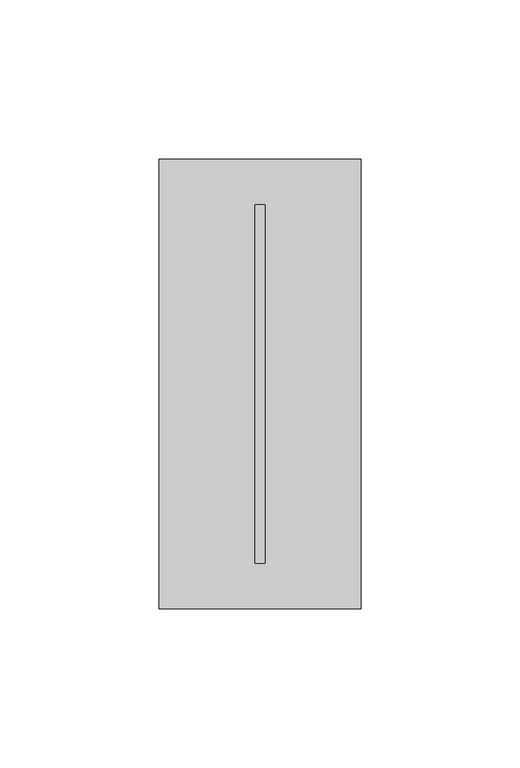
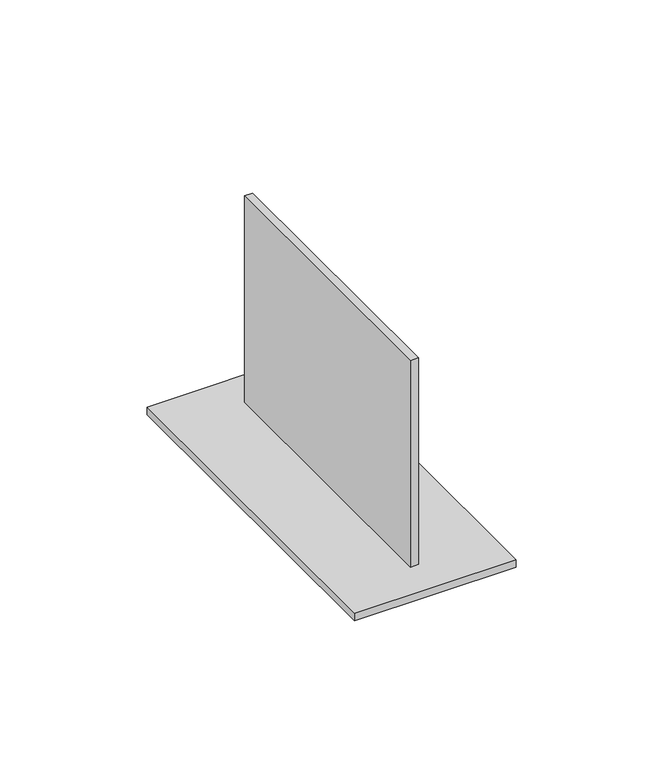
"""IFC4 building model written with IfcOpenShell, lengths in millimetres: proxy geometry, 060523 - W_P_C - Fastenings - Concealed Joist Ties : 060523 - W_P_C - Fastenings - Concealed Joist Ties."""

import ifcopenshell
import ifcopenshell.guid

model = None  # the IFC model being written
_history = None  # IfcOwnerHistory: only IFC2X3 demands one
_inside = {}  # id of a spatial element -> (the spatial element, [elements in it])
_under = {}  # id of a project, library or spatial element -> (it, [spatial elements below it])
_declared = {}  # id of a project -> (the project, [libraries it declares])
_typed = {}  # id of a type object -> (the type object, [elements of that type])
_made_of = {}  # id of a material, layer set ... -> (it, [elements and type objects made of it])


def new_model(schema):
    """Start an empty IFC model of exactly this schema.

    Asked for "IFC4X3", IfcOpenShell would pick the latest addendum, in which some entities
    have other attributes; the version numbers below select the first issue.
    IFC2X3 requires an IfcOwnerHistory on every rooted entity: one is made here for all.
    """
    global model, _history
    if schema == "IFC4X3":
        model = ifcopenshell.file(schema_version=(4, 3, 0, 0))
    else:
        model = ifcopenshell.file(schema=schema)
    _inside.clear()
    _under.clear()
    _declared.clear()
    _typed.clear()
    _made_of.clear()
    _history = None
    if model.schema == "IFC2X3":
        org = make("IfcOrganization", Name="unknown")
        user = make(
            "IfcPersonAndOrganization",
            ThePerson=make("IfcPerson", FamilyName="unknown"),
            TheOrganization=org,
        )
        app = make(
            "IfcApplication",
            ApplicationDeveloper=org,
            Version="unknown",
            ApplicationFullName="unknown",
            ApplicationIdentifier="unknown",
        )
        _history = make(
            "IfcOwnerHistory",
            OwningUser=user,
            OwningApplication=app,
            ChangeAction="ADDED",
            CreationDate=0,
        )
    return model


def make(cls, **values):
    """One entity of the class cls with the attributes given. An attribute that is None is left unset."""
    return model.create_entity(
        cls, **{name: value for name, value in values.items() if value is not None}
    )


def rooted(cls, **values):
    """An entity with a GlobalId (a new one), such as an element, a storey or a relation."""
    return make(cls, GlobalId=ifcopenshell.guid.new(), OwnerHistory=_history, **values)


def si_unit(unit_type, name, prefix=None):
    """IfcSIUnit, for example si_unit("LENGTHUNIT", "METRE", prefix="MILLI")."""
    return make("IfcSIUnit", UnitType=unit_type, Prefix=prefix, Name=name)


def assignment(units):
    """IfcUnitAssignment: the units of a project."""
    return None if units is None else make("IfcUnitAssignment", Units=units)


def point(xyz):
    """IfcCartesianPoint."""
    return None if xyz is None else make("IfcCartesianPoint", Coordinates=xyz)


def direction(xyz):
    """IfcDirection."""
    return None if xyz is None else make("IfcDirection", DirectionRatios=xyz)


def frame(location, z_axis=None, x_axis=None):
    """IfcAxis2Placement3D, a coordinate frame: its origin and axes. An axis left out is left unset."""
    return make(
        "IfcAxis2Placement3D",
        Location=point(location),
        Axis=direction(z_axis),
        RefDirection=direction(x_axis),
    )


def origin():
    """The frame at (0, 0, 0) with its axes left unset."""
    return frame((0.0, 0.0, 0.0))


def origin_with_axes():
    """The frame at (0, 0, 0) with the z axis (0, 0, 1) and the x axis (1, 0, 0) written out."""
    return frame((0.0, 0.0, 0.0), z_axis=(0.0, 0.0, 1.0), x_axis=(1.0, 0.0, 0.0))


def place(relative_to, where):
    """IfcLocalPlacement: puts the frame where relative to a parent placement (None: the world)."""
    return make(
        "IfcLocalPlacement", PlacementRelTo=relative_to, RelativePlacement=where
    )


def context(
    kind, dimensions, precision=None, world=None, true_north=None, identifier=None
):
    """IfcGeometricRepresentationContext, for example the 3D "Model" context."""
    return make(
        "IfcGeometricRepresentationContext",
        ContextIdentifier=identifier,
        ContextType=kind,
        CoordinateSpaceDimension=dimensions,
        Precision=precision,
        WorldCoordinateSystem=world,
        TrueNorth=true_north,
    )


def project(units=None, contexts=None):
    """IfcProject with its units and contexts."""
    return rooted(
        "IfcProject",
        Name="project",
        RepresentationContexts=contexts,
        UnitsInContext=assignment(units),
    )


def spatial(cls, under=None, at=None, **own):
    """A site, building, storey or space (cls), placed at a placement, below another one or the project."""
    s = rooted(cls, ObjectPlacement=at, **own)
    if under is not None:
        _under.setdefault(under.id(), (under, []))[1].append(s)
    return s


def polyline(points):
    """IfcPolyline through the points."""
    return make("IfcPolyline", Points=[point(p) for p in points])


def outline(outer, holes=None, kind="AREA"):
    """IfcArbitraryClosedProfileDef: a profile drawn as a closed curve; with holes, ...WithVoids."""
    if holes is None:
        return make("IfcArbitraryClosedProfileDef", ProfileType=kind, OuterCurve=outer)
    return make(
        "IfcArbitraryProfileDefWithVoids",
        ProfileType=kind,
        OuterCurve=outer,
        InnerCurves=holes,
    )


def extrude(swept, where, along, depth):
    """IfcExtrudedAreaSolid: the profile swept, set in the frame where, extruded along a direction by depth."""
    return make(
        "IfcExtrudedAreaSolid",
        SweptArea=swept,
        Position=where,
        ExtrudedDirection=direction(along),
        Depth=depth,
    )


def shape(context_of_items, identifier, shape_type, items):
    """IfcShapeRepresentation: the items that make up one representation, for example the "Body"."""
    return make(
        "IfcShapeRepresentation",
        ContextOfItems=context_of_items,
        RepresentationIdentifier=identifier,
        RepresentationType=shape_type,
        Items=items,
    )


def source(mapping_origin, context_of_items, identifier, shape_type, items):
    """IfcRepresentationMap: a shape defined once, which mapped items show again and again."""
    return make(
        "IfcRepresentationMap",
        MappingOrigin=mapping_origin,
        MappedRepresentation=shape(context_of_items, identifier, shape_type, items),
    )


def transform(
    local_origin,
    x_axis=None,
    y_axis=None,
    z_axis=None,
    scale=None,
    scale2=None,
    scale3=None,
    uniform=True,
):
    """IfcCartesianTransformationOperator3D, or its non-uniform kind. x_axis, y_axis, z_axis: its Axis1, 2, 3."""
    if uniform:
        return make(
            "IfcCartesianTransformationOperator3D",
            Axis1=direction(x_axis),
            Axis2=direction(y_axis),
            LocalOrigin=point(local_origin),
            Scale=scale,
            Axis3=direction(z_axis),
        )
    return make(
        "IfcCartesianTransformationOperator3DnonUniform",
        Axis1=direction(x_axis),
        Axis2=direction(y_axis),
        LocalOrigin=point(local_origin),
        Scale=scale,
        Axis3=direction(z_axis),
        Scale2=scale2,
        Scale3=scale3,
    )


def mapped(mapping_source, mapping_target):
    """IfcMappedItem: shows the shape of a source again, moved by a transform."""
    return make(
        "IfcMappedItem", MappingSource=mapping_source, MappingTarget=mapping_target
    )


def made_of(thing, what):
    """Note that an element or type object is made of a material, layer set ...; save() writes the relation."""
    if what is not None:
        _made_of.setdefault(what.id(), (what, []))[1].append(thing)
    return thing


def element(
    cls,
    number,
    at=None,
    inside=None,
    cuts=None,
    type_object=None,
    material=None,
    context=None,
    identifier="Body",
    shape_type=None,
    held_by="IfcProductDefinitionShape",
    body=None,
    shapes=None,
    **own,
):
    """One element of the class cls, such as IfcWall. Its Tag is "e" and its number.

    at: its placement. inside: the storey or other place that contains it. cuts: it is an
    opening in that element (IfcRelVoidsElement). A single representation is given by context,
    identifier, shape_type and body (its items); several are given by shapes. held_by: the class
    of the entity that holds the representations. save() writes the other relations.
    """
    e = rooted(cls, Tag="e%d" % number, ObjectPlacement=at, **own)
    if body is not None:
        shapes = [shape(context, identifier, shape_type, body)]
    if shapes is not None:
        e.Representation = make(held_by, Representations=shapes)
    if inside is not None:
        _inside.setdefault(inside.id(), (inside, []))[1].append(e)
    if cuts is not None:
        rooted(
            "IfcRelVoidsElement", RelatingBuildingElement=cuts, RelatedOpeningElement=e
        )
    if type_object is not None:
        _typed.setdefault(type_object.id(), (type_object, []))[1].append(e)
    return made_of(e, material)


def aggregate(whole, parts):
    """IfcRelAggregates: a whole, such as a stair, and the parts it consists of."""
    return rooted("IfcRelAggregates", RelatingObject=whole, RelatedObjects=parts)


def save(model, path):
    """Write the relations noted so far, then the file.

    IfcRelAggregates (storeys below a building ...), IfcRelContainedInSpatialStructure (elements
    in a storey), IfcRelDefinesByType, IfcRelAssociatesMaterial and IfcRelDeclares: one each for
    every whole, place, type object, material and project.
    """
    for whole, parts in _under.values():
        aggregate(whole, parts)
    for where, things in _inside.values():
        rooted(
            "IfcRelContainedInSpatialStructure",
            RelatedElements=things,
            RelatingStructure=where,
        )
    for kind, things in _typed.values():
        rooted("IfcRelDefinesByType", RelatedObjects=things, RelatingType=kind)
    for what, things in _made_of.values():
        rooted("IfcRelAssociatesMaterial", RelatedObjects=things, RelatingMaterial=what)
    for by, libraries in _declared.values():
        rooted("IfcRelDeclares", RelatingContext=by, RelatedDefinitions=libraries)
    model.write(path)


def generic_models_a2696cd2(model_context):
    return source(origin(), model_context, "Body", "SweptSolid", [
        extrude(outline(polyline([(1.5875, 56.35625), (1.5875, -56.35625), (-1.5875, -56.35625), (-1.5875, 56.35625), (1.5875, 56.35625)])), frame((0.0, 0.0, 3.175), z_axis=(0.0, 0.0, 1.0), x_axis=(1.0, 0.0, 0.0)), (0.0, 0.0, 1.0), 85.725),
        extrude(outline(polyline([(31.75, 70.64375), (31.75, -70.64375), (-31.75, -70.64375), (-31.75, 70.64375), (31.75, 70.64375)])), origin_with_axes(), (0.0, 0.0, 1.0), 3.175),
    ])


if __name__ == "__main__":
    model = new_model("IFC4")
    model_context = context("Model", 3, world=origin())
    ifc_project = project(units=[si_unit("LENGTHUNIT", "METRE", prefix="MILLI")], contexts=[model_context])
    site = spatial("IfcSite", under=ifc_project)
    building = spatial("IfcBuilding", under=site)
    placement = place(None, origin())
    generic_models_shape = generic_models_a2696cd2(model_context)
    element("IfcBuildingElementProxy", 1, Name="060523 - W_P_C - Fastenings - Concealed Joist Ties : 060523 - W_P_C - Fastenings - Concealed Joist Ties", ObjectType="060523 - W_P_C - Fastenings - Concealed Joist Ties : 060523 - W_P_C - Fastenings - Concealed Joist Ties", at=placement, inside=building, context=model_context, shape_type="MappedRepresentation", body=[
        mapped(generic_models_shape, transform((0.0, 0.0, 0.0), x_axis=(1.0, 0.0, 0.0), y_axis=(0.0, 1.0, 0.0), z_axis=(0.0, 0.0, 1.0))),
    ])
    save(model, "model.ifc")

# Revit data of these elements
# Type "060523 - W_P_C - Fastenings - Concealed Joist Ties : 060523 - W_P_C - Fastenings - Concealed Joist Ties"
#   OFFSET FROM SURFACE = 0' - 3"
#   H2 = 0' - 4 7/16"
#   H1 = 0' - 5 9/16"
#   GAUGE = 0' - 0 1/8"
#   Default Elevation = 4' - 0"
#   Material = _BEAM HANGER (SEE STRUCT. DWGS)
# Element 1 (IfcBuildingElementProxy, "060523 - W_P_C - Fastenings - Concealed Joist Ties : 060523 - W_P_C - Fastenings - Concealed Joist Ties")
#   Materials on its faces: "_BEAM HANGER (SEE STRUCT. DWGS)"
# Materials
#   "_BEAM HANGER (SEE STRUCT. DWGS)": class "Generic", colour RGB 191 191 191, transparency 0, Cost = 0
